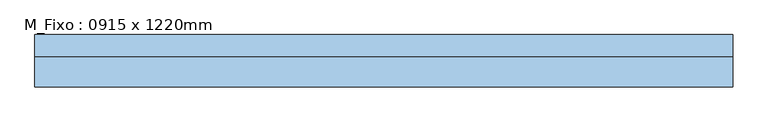
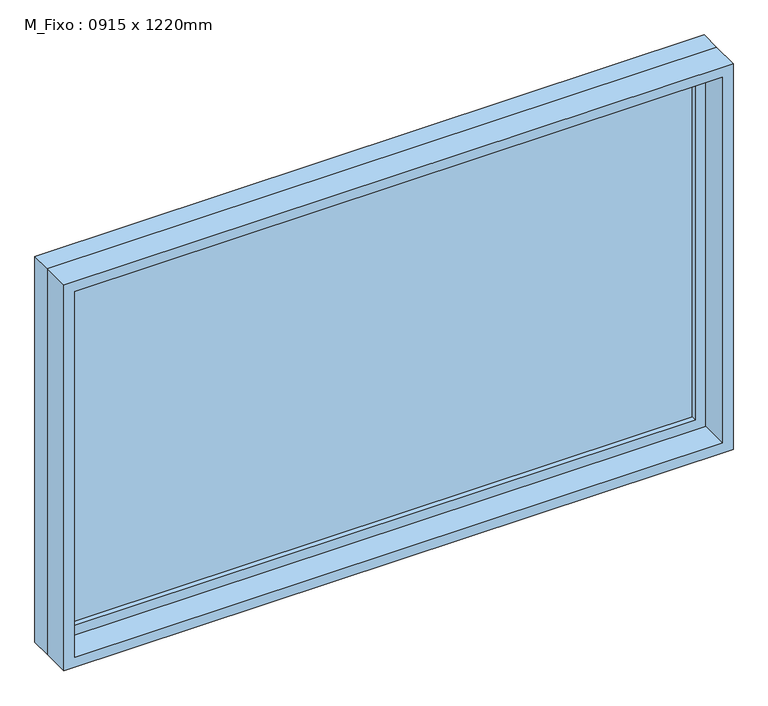
"""IFC4 building model written with IfcOpenShell, lengths in millimetres: window geometry, M_Fixo : 0915 x 1220mm."""

from ifc_helpers import new_model, si_unit, frame, origin, place, context, project, spatial, polyline, outline, extrude, source, transform, mapped, element, save


def m_fixo_0915_x_1220mm_8e554ddc(model_context):
    return source(origin(), model_context, "Body", "SweptSolid", [
        extrude(outline(polyline([(-937.0, 53.0), (937.0, 53.0), (937.0, 41.0), (-937.0, 41.0), (-937.0, 53.0)])), frame((0.0, 0.0, 978.0), z_axis=(0.0, 0.0, 1.0), x_axis=(1.0, 0.0, 0.0)), (0.0, 0.0, 1.0), 1094.0),
        extrude(outline(polyline([(2116.0, -981.0), (934.0, -981.0), (934.0, 981.0), (2116.0, 981.0), (2116.0, -981.0)]), holes=[polyline([(2072.0, -937.0), (2072.0, 937.0), (978.0, 937.0), (978.0, -937.0), (2072.0, -937.0)])]), frame((0.0, 25.0, 0.0), z_axis=(0.0, 1.0, 0.0), x_axis=(0.0, 0.0, 1.0)), (0.0, 0.0, 1.0), 44.0),
        extrude(outline(polyline([(2135.0, -1000.0), (915.0, -1000.0), (915.0, 1000.0), (2135.0, 1000.0), (2135.0, -1000.0)]), holes=[polyline([(2116.0, -981.0), (2116.0, 981.0), (934.0, 981.0), (934.0, -981.0), (2116.0, -981.0)])]), frame((0.0, 25.0, 0.0), z_axis=(0.0, 1.0, 0.0), x_axis=(0.0, 0.0, 1.0)), (0.0, 0.0, 1.0), 63.0),
        extrude(outline(polyline([(2135.0, -1000.0), (915.0, -1000.0), (915.0, 1000.0), (2135.0, 1000.0), (2135.0, -1000.0)]), holes=[polyline([(2103.0, -968.0), (2103.0, 968.0), (947.0, 968.0), (947.0, -968.0), (2103.0, -968.0)])]), frame((0.0, -62.0, 0.0), z_axis=(0.0, 1.0, 0.0), x_axis=(0.0, 0.0, 1.0)), (0.0, 0.0, 1.0), 87.0),
    ])


if __name__ == "__main__":
    model = new_model("IFC4")
    model_context = context("Model", 3, world=origin())
    ifc_project = project(units=[si_unit("LENGTHUNIT", "METRE", prefix="MILLI")], contexts=[model_context])
    site = spatial("IfcSite", under=ifc_project)
    building = spatial("IfcBuilding", under=site)
    placement = place(None, origin())
    m_fixo_0915_x_1220mm_shape = m_fixo_0915_x_1220mm_8e554ddc(model_context)
    element("IfcWindow", 1, ObjectType="M_Fixo : 0915 x 1220mm", at=placement, inside=building, context=model_context, shape_type="MappedRepresentation", body=[
        mapped(m_fixo_0915_x_1220mm_shape, transform((0.0, 0.0, 0.0), x_axis=(1.0, 0.0, 0.0), y_axis=(0.0, 1.0, 0.0), z_axis=(0.0, 0.0, 1.0))),
    ])
    save(model, "model.ifc")

# Revit data of these elements
# Type "M_Fixo : 0915 x 1220mm"
#   Type Mark = "15"
#   Construction Type Id = "GSP4R"
#   Analytic Construction = "Vidraça única Pilkington 1/8 pol"
#   Visual Light Transmittance = 0.9
#   Thermal Resistance (R) = 0.271106 (m²·K)/W
#   Solar Heat Gain Coefficient = 0.78
#   Heat Transfer Coefficient (U) = 3.6886 W/(m²·K)
#   Height = 1.22 m
#   Altura-padrão do peitoril = 0.915 m
#   Width = 2.00 m
#   Janela aplicada = 0.019 m
#   Define Thermal Properties by = 1
#   Material da estrutura externa = Caixilho
#   Material da estrutura interna = Caixilho
#   Material do painel de vidro = Vidro
#   Caixilho = Caixilho
#   Wall Closure = (empty or 0)
# Element 1 (IfcWindow, "M_Fixo : 0915 x 1220mm")
#   Materials on its faces: "Caixilho", "Vidro"
# Materials
#   "Caixilho": class "Madeira", colour RGB 224 178 126, transparency 0, Cost = 0
#   "Vidro": class "Vidro", colour RGB 0 128 192, transparency 0.9, Description = "Vidro de sílica", Cost = 0
